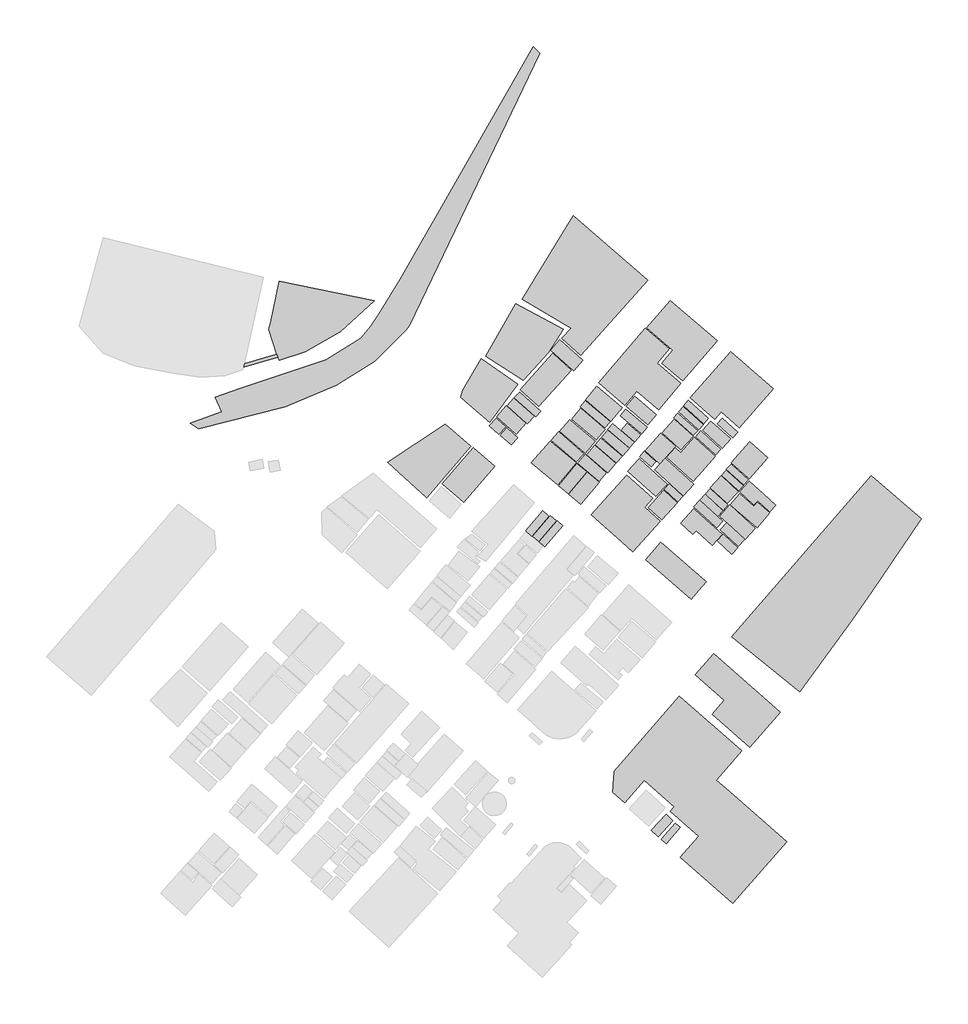
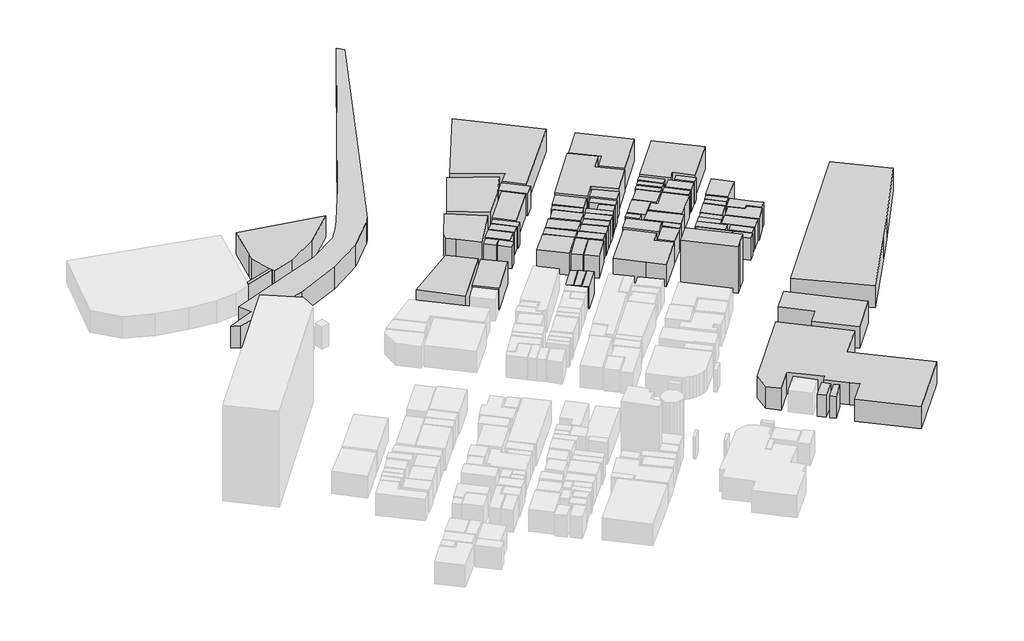
# Not in any storey, part 3 of 3: 71 proxies.
"""IFC4 building model written with IfcOpenShell, lengths in millimetres."""

from ifc_helpers import new_model, si_unit, origin, origin_with_axes, place, context, project, spatial, polyline, outline, extrude, element, save

model = new_model("IFC4")

# Units and contexts
model_context = context("Model", 3, world=origin())
ifc_project = project(units=[si_unit("LENGTHUNIT", "METRE", prefix="MILLI")], contexts=[model_context])

# Site, building
site = spatial("IfcSite", under=ifc_project)
building = spatial("IfcBuilding", under=site)

# Proxies
placement = place(None, origin())
element("IfcBuildingElementProxy", 1, Name="Mass", at=placement, inside=building, context=model_context, shape_type="SweptSolid", body=[
    extrude(outline(polyline([(247570.5222327, 178356.6623379), (255926.1515654, 187930.5455225), (280776.244849, 166225.2958414), (276476.4831621, 161299.3605912), (272420.6155188, 156651.4126569), (247570.5222327, 178356.6623379)])), origin_with_axes(), (0.0, 0.0, 1.0), 32000.0),
])
element("IfcBuildingElementProxy", 2, Name="Mass", at=placement, inside=building, context=model_context, shape_type="SweptSolid", body=[
    extrude(outline(polyline([(258708.3503039, 38751.4319358), (262511.2907886, 35271.0307322), (254408.5886169, 26397.6755858), (250596.6150174, 29878.0767893), (258708.3503039, 38751.4319358)])), origin_with_axes(), (0.0, 0.0, 1.0), 15000.0),
])
element("IfcBuildingElementProxy", 3, Name="Mass", at=placement, inside=building, context=model_context, shape_type="SweptSolid", body=[
    extrude(outline(polyline([(263766.8934663, 33847.7356711), (266413.5955132, 31557.1201823), (258708.3503039, 22661.5260503), (256061.6482569, 24952.1415391), (263766.8934663, 33847.7356711)])), origin_with_axes(), (0.0, 0.0, 1.0), 15000.0),
])
element("IfcBuildingElementProxy", 4, Name="Mass", at=placement, inside=building, context=model_context, shape_type="SweptSolid", body=[
    extrude(outline(polyline([(288409.2251578, 194680.0775697), (291896.0066931, 198527.4220315), (301913.7287781, 189453.9160172), (298426.9472428, 185595.4520625), (288409.2251578, 194680.0775697)])), origin_with_axes(), (0.0, 0.0, 1.0), 15000.0),
])
element("IfcBuildingElementProxy", 5, Name="Mass", at=placement, inside=building, context=model_context, shape_type="SweptSolid", body=[
    extrude(outline(polyline([(293955.5564102, 208390.4120248), (299230.8942796, 214483.894005), (306909.0401522, 207712.1229722), (308869.2256268, 209891.5435347), (315571.795317, 204165.0048127), (308643.3978076, 195803.1463285), (293955.5564102, 208390.4120248)])), origin_with_axes(), (0.0, 0.0, 1.0), 15000.0),
])
element("IfcBuildingElementProxy", 6, Name="Mass", at=placement, inside=building, context=model_context, shape_type="SweptSolid", body=[
    extrude(outline(polyline([(288056.9337594, 202308.0495374), (293585.1987872, 208412.6510104), (307613.6229491, 195703.0708949), (302085.3579212, 189598.4694219), (288056.9337594, 202308.0495374)])), origin_with_axes(), (0.0, 0.0, 1.0), 15000.0),
])
element("IfcBuildingElementProxy", 7, Name="Mass", at=placement, inside=building, context=model_context, shape_type="SweptSolid", body=[
    extrude(outline(polyline([(266016.138551, 103344.5648239), (300152.2717833, 73566.5634681), (286159.9800731, 57532.2550459), (291381.1192664, 52984.3825467), (324812.6697019, 23806.8337947), (295283.4239911, -10040.9018756), (266521.992868, 15055.7930682), (276621.0129658, 26631.1849313), (272176.7214726, 30511.8878715), (260912.4298247, 40330.3998944), (263188.7742487, 42943.4806703), (246667.2109559, 57354.3431635), (236026.2040895, 45156.2597103), (229459.1310908, 50882.798433), (230190.813227, 62280.2784138), (266016.138551, 103344.5648239)])), origin_with_axes(), (0.0, 0.0, 1.0), 15000.0),
])
element("IfcBuildingElementProxy", 8, Name="Mass", at=placement, inside=building, context=model_context, shape_type="SweptSolid", body=[
    extrude(outline(polyline([(286801.3310816, 188664.4320382), (290098.4172494, 192300.5061393), (298155.9538572, 185006.1189515), (294858.8676895, 181370.0448504), (286801.3310816, 188664.4320382)])), origin_with_axes(), (0.0, 0.0, 1.0), 15000.0),
])
element("IfcBuildingElementProxy", 9, Name="Mass", at=placement, inside=building, context=model_context, shape_type="SweptSolid", body=[
    extrude(outline(polyline([(371125.4389763, 224313.5255207), (398784.8303376, 200773.5595499), (371414.4985838, 160754.5054506), (360818.6572812, 145454.0835441), (332129.4910613, 105879.809151), (294768.5365618, 136180.4266618), (371125.4389763, 224313.5255207)])), origin_with_axes(), (0.0, 0.0, 1.0), 15000.0),
])
element("IfcBuildingElementProxy", 10, Name="Mass", at=placement, inside=building, context=model_context, shape_type="SweptSolid", body=[
    extrude(outline(polyline([(45355.2593164, 291052.7204921), (45843.0474089, 289418.1550711), (26927.7092252, 283791.6917827), (27442.5966544, 285726.483506), (45355.2593164, 291052.7204921)])), origin_with_axes(), (0.0, 0.0, 1.0), 15000.0),
])
element("IfcBuildingElementProxy", 11, Name="Mass", at=placement, inside=building, context=model_context, shape_type="SweptSolid", body=[
    extrude(outline(polyline([(321479.4510826, 94793.6749646), (304650.7619527, 75568.0721482), (284028.1654554, 93615.0087426), (290640.4040154, 101176.2637543), (274678.8937157, 115153.4660333), (284895.3442831, 126817.8138387), (321479.4510826, 94793.6749646)])), origin_with_axes(), (0.0, 0.0, 1.0), 15000.0),
])
element("IfcBuildingElementProxy", 12, Name="Mass", at=placement, inside=building, context=model_context, shape_type="SweptSolid", body=[
    extrude(outline(polyline([(157465.2221542, 288561.9541354), (177428.401421, 274562.5128708), (162045.010339, 253624.5081838), (150672.3213364, 263331.8252796), (146237.0629554, 267490.5155365), (147212.6391378, 271371.2184759), (157465.2221542, 288561.9541354)])), origin_with_axes(), (0.0, 0.0, 1.0), 15000.0),
])
element("IfcBuildingElementProxy", 13, Name="Mass", at=placement, inside=building, context=model_context, shape_type="SweptSolid", body=[
    extrude(outline(polyline([(41913.6433449, 308488.0849906), (46646.9944457, 331171.8500257), (98713.8565671, 320363.703156), (80105.6442205, 303306.4014085), (60720.5841739, 292442.6570756), (46728.2924611, 287872.54559), (45843.0474089, 289418.1550711), (45355.2593164, 291052.7204921), (40929.0340502, 304629.621036), (41913.6433449, 308488.0849906)])), origin_with_axes(), (0.0, 0.0, 1.0), 15000.0),
])
element("IfcBuildingElementProxy", 14, Name="Mass", at=placement, inside=building, context=model_context, shape_type="SweptSolid", body=[
    extrude(outline(polyline([(175314.6530278, 266967.8993815), (186371.183081, 257071.5509098), (182640.5074995, 252912.8606537), (171583.9774437, 262798.0896318), (175314.6530278, 266967.8993815)])), origin_with_axes(), (0.0, 0.0, 1.0), 15000.0),
])
element("IfcBuildingElementProxy", 15, Name="Mass", at=placement, inside=building, context=model_context, shape_type="SweptSolid", body=[
    extrude(outline(polyline([(236640.4557587, 260996.7318204), (248347.3699327, 251078.1443639), (245312.2440357, 247497.667726), (233605.3298618, 257427.3746753), (236640.4557587, 260996.7318204)])), origin_with_axes(), (0.0, 0.0, 1.0), 15000.0),
])
element("IfcBuildingElementProxy", 16, Name="Mass", at=placement, inside=building, context=model_context, shape_type="SweptSolid", body=[
    extrude(outline(polyline([(199803.4218007, 248465.0635873), (213461.4883396, 236578.3259291), (209486.9187118, 231997.0949516), (195819.8190607, 243883.8326097), (199803.4218007, 248465.0635873)])), origin_with_axes(), (0.0, 0.0, 1.0), 15000.0),
])
element("IfcBuildingElementProxy", 17, Name="Mass", at=placement, inside=building, context=model_context, shape_type="SweptSolid", body=[
    extrude(outline(polyline([(178458.176277, 270237.0302243), (190029.593762, 259873.6630616), (187184.1632327, 256693.4881595), (175603.7126354, 267045.7358294), (178458.176277, 270237.0302243)])), origin_with_axes(), (0.0, 0.0, 1.0), 15000.0),
])
element("IfcBuildingElementProxy", 18, Name="Mass", at=placement, inside=building, context=model_context, shape_type="SweptSolid", body=[
    extrude(outline(polyline([(237408.2703439, 253190.8479696), (244743.1579304, 246975.0515702), (241464.1379872, 243116.5876156), (234129.2504033, 249332.384015), (237408.2703439, 253190.8479696)])), origin_with_axes(), (0.0, 0.0, 1.0), 15000.0),
])
element("IfcBuildingElementProxy", 19, Name="Mass", at=placement, inside=building, context=model_context, shape_type="SweptSolid", body=[
    extrude(outline(polyline([(220805.4090383, 273361.6076632), (234608.005381, 261652.7818874), (228402.256893, 254325.036222), (214599.6605503, 266033.861997), (220805.4090383, 273361.6076632)])), origin_with_axes(), (0.0, 0.0, 1.0), 15000.0),
])
element("IfcBuildingElementProxy", 20, Name="Mass", at=placement, inside=building, context=model_context, shape_type="SweptSolid", body=[
    extrude(outline(polyline([(214491.2631982, 265411.1704084), (228022.8661552, 253935.8539781), (225222.6011923, 250622.2451641), (211681.9651204, 262108.6810864), (214491.2631982, 265411.1704084)])), origin_with_axes(), (0.0, 0.0, 1.0), 15000.0),
])
element("IfcBuildingElementProxy", 21, Name="Mass", at=placement, inside=building, context=model_context, shape_type="SweptSolid", body=[
    extrude(outline(polyline([(171051.0237899, 262709.133691), (181782.361784, 253101.8920288), (176507.0239146, 247208.5609165), (165775.6859206, 256815.8025787), (171051.0237899, 262709.133691)])), origin_with_axes(), (0.0, 0.0, 1.0), 15000.0),
])
element("IfcBuildingElementProxy", 22, Name="Mass", at=placement, inside=building, context=model_context, shape_type="SweptSolid", body=[
    extrude(outline(polyline([(207029.9120325, 255370.268532), (212061.3558556, 261296.9581227), (225394.2303353, 249988.4340827), (220371.8196245, 244061.7444921), (207029.9120325, 255370.268532)])), origin_with_axes(), (0.0, 0.0, 1.0), 15000.0),
])
element("IfcBuildingElementProxy", 23, Name="Mass", at=placement, inside=building, context=model_context, shape_type="SweptSolid", body=[
    extrude(outline(polyline([(247236.2970613, 238123.9354094), (255890.0191138, 247797.8940275), (263911.4232701, 240614.7017661), (255266.7343298, 230951.8626407), (247236.2970613, 238123.9354094)])), origin_with_axes(), (0.0, 0.0, 1.0), 15000.0),
])
element("IfcBuildingElementProxy", 24, Name="Mass", at=placement, inside=building, context=model_context, shape_type="SweptSolid", body=[
    extrude(outline(polyline([(214355.7665041, 236055.7097741), (226008.4820045, 226159.3613024), (222033.9123767, 221478.0548905), (210381.1968788, 231374.4033622), (214355.7665041, 236055.7097741)])), origin_with_axes(), (0.0, 0.0, 1.0), 15000.0),
])
element("IfcBuildingElementProxy", 25, Name="Mass", at=placement, inside=building, context=model_context, shape_type="SweptSolid", body=[
    extrude(outline(polyline([(288942.1788116, 259417.7638618), (285500.5628401, 255503.702444), (272122.5227965, 267268.125683), (294280.7484718, 292476.0155532), (317595.2125825, 271982.7905725), (298878.6028811, 250688.9621201), (288942.1788116, 259417.7638618)])), origin_with_axes(), (0.0, 0.0, 1.0), 15000.0),
])
element("IfcBuildingElementProxy", 26, Name="Mass", at=placement, inside=building, context=model_context, shape_type="SweptSolid", body=[
    extrude(outline(polyline([(260912.4298247, 320497.137068), (286683.9006146, 298558.3780406), (267822.7611095, 276397.2291605), (256441.0389947, 286082.3072714), (262502.2576763, 293209.9020689), (248112.5090013, 305452.4634925), (260912.4298247, 320497.137068)])), origin_with_axes(), (0.0, 0.0, 1.0), 15000.0),
])
element("IfcBuildingElementProxy", 27, Name="Mass", at=placement, inside=building, context=model_context, shape_type="SweptSolid", body=[
    extrude(outline(polyline([(259042.5754778, 234465.6223227), (263703.661678, 239680.6643824), (266684.5888963, 237011.9861434), (274164.0062865, 245373.8446268), (285717.357547, 235032.7164489), (278237.9401568, 226681.9774575), (273567.8208444, 221466.9353985), (259042.5754778, 234465.6223227)])), origin_with_axes(), (0.0, 0.0, 1.0), 15000.0),
])
element("IfcBuildingElementProxy", 28, Name="Mass", at=placement, inside=building, context=model_context, shape_type="SweptSolid", body=[
    extrude(outline(polyline([(242530.0452973, 270815.2438433), (236017.1709747, 263142.7939044), (221690.6540905, 275318.6383721), (247191.1314975, 305330.1490734), (260524.0059747, 293999.3860486), (253830.4693967, 286115.665749), (266919.4498303, 275007.2925778), (254625.3833238, 260529.7131286), (242530.0452973, 270815.2438433)])), origin_with_axes(), (0.0, 0.0, 1.0), 15000.0),
])
element("IfcBuildingElementProxy", 29, Name="Mass", at=placement, inside=building, context=model_context, shape_type="SweptSolid", body=[
    extrude(outline(polyline([(217788.3493659, 203008.5775755), (237236.6412034, 224747.1857341), (251454.7607328, 212026.4861259), (246947.2374512, 206989.3559493), (255474.4959245, 199361.3839816), (240533.7273711, 182659.9059996), (232006.4688979, 190287.8779672), (217788.3493659, 203008.5775755)])), origin_with_axes(), (0.0, 0.0, 1.0), 15000.0),
])
element("IfcBuildingElementProxy", 30, Name="Mass", at=placement, inside=building, context=model_context, shape_type="SweptSolid", body=[
    extrude(outline(polyline([(257660.5092208, 216885.7044202), (260352.3768316, 219899.0869327), (267958.2578011, 213093.9574215), (265266.3901903, 210080.5749098), (257660.5092208, 216885.7044202)])), origin_with_axes(), (0.0, 0.0, 1.0), 15000.0),
])
element("IfcBuildingElementProxy", 31, Name="Mass", at=placement, inside=building, context=model_context, shape_type="SweptSolid", body=[
    extrude(outline(polyline([(252394.2044637, 227560.4173779), (258157.330423, 234009.7231236), (273965.2778066, 219865.7284543), (268202.1518473, 213416.4227094), (252394.2044637, 227560.4173779)])), origin_with_axes(), (0.0, 0.0, 1.0), 15000.0),
])
element("IfcBuildingElementProxy", 32, Name="Mass", at=placement, inside=building, context=model_context, shape_type="SweptSolid", body=[
    extrude(outline(polyline([(237814.760421, 226748.6944142), (243939.2108936, 233587.1824022), (259286.4695215, 219865.7284543), (253162.0190515, 213016.1209735), (237814.760421, 226748.6944142)])), origin_with_axes(), (0.0, 0.0, 1.0), 15000.0),
])
element("IfcBuildingElementProxy", 33, Name="Mass", at=placement, inside=building, context=model_context, shape_type="SweptSolid", body=[
    extrude(outline(polyline([(176416.692787, 318662.4207782), (202441.0907354, 304763.054948), (194022.2296144, 291819.9654862), (180454.4942031, 276842.0088675), (159849.9639304, 289985.2491965), (176416.692787, 318662.4207782)])), origin_with_axes(), (0.0, 0.0, 1.0), 15000.0),
])
element("IfcBuildingElementProxy", 34, Name="Mass", at=placement, inside=building, context=model_context, shape_type="SweptSolid", body=[
    extrude(outline(polyline([(277686.9202759, 248943.2017719), (288761.5165562, 239046.853301), (285979.3178178, 235933.395355), (274913.7546497, 245840.8633186), (277686.9202759, 248943.2017719)])), origin_with_axes(), (0.0, 0.0, 1.0), 15000.0),
])
element("IfcBuildingElementProxy", 35, Name="Mass", at=placement, inside=building, context=model_context, shape_type="SweptSolid", body=[
    extrude(outline(polyline([(270975.3174735, 265733.6356955), (281896.3508352, 255959.601643), (279267.7150128, 253024.05558), (268346.6816511, 262798.0896318), (270975.3174735, 265733.6356955)])), origin_with_axes(), (0.0, 0.0, 1.0), 15000.0),
])
element("IfcBuildingElementProxy", 36, Name="Mass", at=placement, inside=building, context=model_context, shape_type="SweptSolid", body=[
    extrude(outline(polyline([(223325.647506, 245485.0395531), (226667.8992376, 249421.3399565), (238456.1114295, 239424.9160513), (235113.8596954, 235488.6156479), (223325.647506, 245485.0395531)])), origin_with_axes(), (0.0, 0.0, 1.0), 15000.0),
])
element("IfcBuildingElementProxy", 37, Name="Mass", at=placement, inside=building, context=model_context, shape_type="SweptSolid", body=[
    extrude(outline(polyline([(205394.918617, 214194.7871955), (215484.9056051, 226337.2731856), (222061.011716, 220877.6022867), (211961.9916156, 208735.1162975), (205394.918617, 214194.7871955)])), origin_with_axes(), (0.0, 0.0, 1.0), 15000.0),
])
element("IfcBuildingElementProxy", 38, Name="Mass", at=placement, inside=building, context=model_context, shape_type="SweptSolid", body=[
    extrude(outline(polyline([(244210.2042766, 234910.4020297), (246721.409632, 237712.5141807), (252990.3899084, 232108.2898779), (250479.1845529, 229306.1777269), (244210.2042766, 234910.4020297)])), origin_with_axes(), (0.0, 0.0, 1.0), 15000.0),
])
element("IfcBuildingElementProxy", 39, Name="Mass", at=placement, inside=building, context=model_context, shape_type="SweptSolid", body=[
    extrude(outline(polyline([(219865.9653075, 241315.2298042), (223045.6210082, 245062.4988325), (234644.1378325, 235221.747824), (231473.5152415, 231485.5982885), (219865.9653075, 241315.2298042)])), origin_with_axes(), (0.0, 0.0, 1.0), 15000.0),
])
element("IfcBuildingElementProxy", 40, Name="Mass", at=placement, inside=building, context=model_context, shape_type="SweptSolid", body=[
    extrude(outline(polyline([(268175.052508, 262130.920072), (279150.2845483, 252312.4080491), (276684.2447567, 249554.7738685), (265709.0127164, 259373.2858914), (268175.052508, 262130.920072)])), origin_with_axes(), (0.0, 0.0, 1.0), 15000.0),
])
element("IfcBuildingElementProxy", 41, Name="Mass", at=placement, inside=building, context=model_context, shape_type="SweptSolid", body=[
    extrude(outline(polyline([(200381.5410184, 248687.4534408), (205828.5080308, 255103.4007081), (219874.9984197, 243194.4240644), (214428.0314072, 236778.4767971), (200381.5410184, 248687.4534408)])), origin_with_axes(), (0.0, 0.0, 1.0), 15000.0),
])
element("IfcBuildingElementProxy", 42, Name="Mass", at=placement, inside=building, context=model_context, shape_type="SweptSolid", body=[
    extrude(outline(polyline([(165513.7256498, 255970.7211358), (170807.1297437, 251233.8172607), (167058.3879376, 247041.7685262), (161764.9838411, 251789.7918941), (165513.7256498, 255970.7211358)])), origin_with_axes(), (0.0, 0.0, 1.0), 15000.0),
])
element("IfcBuildingElementProxy", 43, Name="Mass", at=placement, inside=building, context=model_context, shape_type="SweptSolid", body=[
    extrude(outline(polyline([(199767.2893492, 218953.9300562), (209766.9452071, 230951.8626407), (215141.6473189, 226470.7070975), (205141.9914585, 214472.7745122), (199767.2893492, 218953.9300562)])), origin_with_axes(), (0.0, 0.0, 1.0), 15000.0),
])
element("IfcBuildingElementProxy", 44, Name="Mass", at=placement, inside=building, context=model_context, shape_type="SweptSolid", body=[
    extrude(outline(polyline([(226685.9654646, 249855.0001708), (229368.7999632, 253012.9360873), (241346.7075227, 242860.8392845), (238663.8730242, 239691.7838752), (226685.9654646, 249855.0001708)])), origin_with_axes(), (0.0, 0.0, 1.0), 15000.0),
])
element("IfcBuildingElementProxy", 45, Name="Mass", at=placement, inside=building, context=model_context, shape_type="SweptSolid", body=[
    extrude(outline(polyline([(241608.6677935, 267990.8927059), (253414.94621, 257983.3493087), (248708.6944459, 252434.7224691), (236902.4160295, 262442.2658671), (241608.6677935, 267990.8927059)])), origin_with_axes(), (0.0, 0.0, 1.0), 15000.0),
])
element("IfcBuildingElementProxy", 46, Name="Mass", at=placement, inside=building, context=model_context, shape_type="SweptSolid", body=[
    extrude(outline(polyline([(265266.3901903, 258717.2358244), (276006.7612966, 249109.9941622), (273730.4168726, 246563.6303416), (262990.0457663, 256181.9914965), (265266.3901903, 258717.2358244)])), origin_with_axes(), (0.0, 0.0, 1.0), 15000.0),
])
element("IfcBuildingElementProxy", 47, Name="Mass", at=placement, inside=building, context=model_context, shape_type="SweptSolid", body=[
    extrude(outline(polyline([(200562.2032737, 298903.0823133), (213109.1969412, 287683.5142149), (207969.3557633, 281934.7365073), (195422.3620984, 293165.4240985), (200562.2032737, 298903.0823133)])), origin_with_axes(), (0.0, 0.0, 1.0), 15000.0),
])
element("IfcBuildingElementProxy", 48, Name="Mass", at=placement, inside=building, context=model_context, shape_type="SweptSolid", body=[
    extrude(outline(polyline([(215123.5810919, 235900.0368766), (219513.673909, 241070.6009659), (231039.9258277, 231307.6864062), (226649.8330131, 226126.0028249), (215123.5810919, 235900.0368766)])), origin_with_axes(), (0.0, 0.0, 1.0), 15000.0),
])
element("IfcBuildingElementProxy", 49, Name="Mass", at=placement, inside=building, context=model_context, shape_type="SweptSolid", body=[
    extrude(outline(polyline([(263188.7742487, 255303.551576), (273558.7877295, 246029.8946938), (266910.416718, 238590.9541012), (256540.4032346, 247875.7304763), (263188.7742487, 255303.551576)])), origin_with_axes(), (0.0, 0.0, 1.0), 15000.0),
])
element("IfcBuildingElementProxy", 50, Name="Mass", at=placement, inside=building, context=model_context, shape_type="SweptSolid", body=[
    extrude(outline(polyline([(289565.4635956, 255881.765195), (298065.6227295, 248276.0322121), (295364.7220065, 245262.6497004), (286864.56287, 252868.3826825), (289565.4635956, 255881.765195)])), origin_with_axes(), (0.0, 0.0, 1.0), 15000.0),
])
element("IfcBuildingElementProxy", 51, Name="Mass", at=placement, inside=building, context=model_context, shape_type="SweptSolid", body=[
    extrude(outline(polyline([(249042.9196199, 206900.4000077), (257452.7476261, 216307.490802), (264868.933228, 209669.1536811), (256459.1052192, 200273.1823797), (249042.9196199, 206900.4000077)])), origin_with_axes(), (0.0, 0.0, 1.0), 15000.0),
])
element("IfcBuildingElementProxy", 52, Name="Mass", at=placement, inside=building, context=model_context, shape_type="SweptSolid", body=[
    extrude(outline(polyline([(195332.0309707, 243361.2164547), (209351.4220203, 231652.3906789), (199198.2032438, 219498.7851968), (184781.355232, 231641.2711861), (195332.0309707, 243361.2164547)])), origin_with_axes(), (0.0, 0.0, 1.0), 15000.0),
])
element("IfcBuildingElementProxy", 53, Name="Mass", at=placement, inside=building, context=model_context, shape_type="SweptSolid", body=[
    extrude(outline(polyline([(283323.582656, 254369.5141924), (294253.6491325, 244584.3606479), (289673.8609478, 239458.2745297), (278734.761359, 249243.4280742), (283323.582656, 254369.5141924)])), origin_with_axes(), (0.0, 0.0, 1.0), 15000.0),
])
element("IfcBuildingElementProxy", 54, Name="Mass", at=placement, inside=building, context=model_context, shape_type="SweptSolid", body=[
    extrude(outline(polyline([(178674.9709839, 271682.564271), (196470.2031814, 291564.2171551), (206840.2166649, 282279.44078), (189044.9844673, 262397.7878959), (178674.9709839, 271682.564271)])), origin_with_axes(), (0.0, 0.0, 1.0), 15000.0),
])
element("IfcBuildingElementProxy", 55, Name="Mass", at=placement, inside=building, context=model_context, shape_type="SweptSolid", body=[
    extrude(outline(polyline([(289240.2715339, 224658.2297926), (291778.5762287, 227449.2224516), (301109.7817413, 218998.4080266), (298571.4770465, 216196.2958756), (289240.2715339, 224658.2297926)])), origin_with_axes(), (0.0, 0.0, 1.0), 15000.0),
])
element("IfcBuildingElementProxy", 56, Name="Mass", at=placement, inside=building, context=model_context, shape_type="SweptSolid", body=[
    extrude(outline(polyline([(185720.7989603, 191288.6323069), (195332.0309707, 202530.4393909), (198475.5542199, 199850.6416582), (188864.322212, 188597.7150823), (185720.7989603, 191288.6323069)])), origin_with_axes(), (0.0, 0.0, 1.0), 15000.0),
])
element("IfcBuildingElementProxy", 57, Name="Mass", at=placement, inside=building, context=model_context, shape_type="SweptSolid", body=[
    extrude(outline(polyline([(181782.361784, 194168.5809067), (191122.6004089, 205087.9227036), (194455.8190282, 202241.3325814), (185115.5804033, 191321.9907845), (181782.361784, 194168.5809067)])), origin_with_axes(), (0.0, 0.0, 1.0), 15000.0),
])
element("IfcBuildingElementProxy", 58, Name="Mass", at=placement, inside=building, context=model_context, shape_type="SweptSolid", body=[
    extrude(outline(polyline([(179894.4412126, 321264.3820621), (207897.0908602, 367032.2138689), (248699.6613337, 331672.227196), (211862.6273757, 290596.821293), (201546.8125684, 299903.8366529), (206641.4881824, 305407.9855221), (179894.4412126, 321264.3820621)])), origin_with_axes(), (0.0, 0.0, 1.0), 15000.0),
])
element("IfcBuildingElementProxy", 59, Name="Mass", at=placement, inside=building, context=model_context, shape_type="SweptSolid", body=[
    extrude(outline(polyline([(308950.5236422, 210614.3105576), (306954.205716, 208412.6510104), (299113.4638126, 215518.006823), (304325.5698936, 221277.9040226), (312175.3449067, 214172.5482107), (318814.6828086, 208156.9026785), (315589.8615415, 204598.6650261), (308950.5236422, 210614.3105576)])), origin_with_axes(), (0.0, 0.0, 1.0), 15000.0),
])
element("IfcBuildingElementProxy", 60, Name="Mass", at=placement, inside=building, context=model_context, shape_type="SweptSolid", body=[
    extrude(outline(polyline([(274010.4433705, 206311.0668967), (280631.7150452, 200306.5408581), (289520.2980317, 192256.0281689), (284127.5296954, 186307.0995935), (275247.9798237, 194357.6122826), (273405.2248135, 192322.7451249), (266774.9200265, 198327.2711636), (274010.4433705, 206311.0668967)])), origin_with_axes(), (0.0, 0.0, 1.0), 15000.0),
])
element("IfcBuildingElementProxy", 61, Name="Mass", at=placement, inside=building, context=model_context, shape_type="SweptSolid", body=[
    extrude(outline(polyline([(273802.6817758, 207456.3746411), (277090.7348313, 211081.3292494), (289890.6556547, 199483.6984008), (286602.6025992, 195858.7437917), (273802.6817758, 207456.3746411)])), origin_with_axes(), (0.0, 0.0, 1.0), 15000.0),
])
element("IfcBuildingElementProxy", 62, Name="Mass", at=placement, inside=building, context=model_context, shape_type="SweptSolid", body=[
    extrude(outline(polyline([(291868.9073563, 227882.8826658), (294371.0795995, 230640.5168464), (303738.4175612, 222145.2244511), (301245.2784328, 219387.5902697), (291868.9073563, 227882.8826658)])), origin_with_axes(), (0.0, 0.0, 1.0), 15000.0),
])
element("IfcBuildingElementProxy", 63, Name="Mass", at=placement, inside=building, context=model_context, shape_type="SweptSolid", body=[
    extrude(outline(polyline([(282953.2250331, 217741.9053558), (288878.9470232, 224280.1670423), (298291.4505487, 215751.5161686), (292365.7285585, 209213.2544821), (282953.2250331, 217741.9053558)])), origin_with_axes(), (0.0, 0.0, 1.0), 15000.0),
])
element("IfcBuildingElementProxy", 64, Name="Mass", at=placement, inside=building, context=model_context, shape_type="SweptSolid", body=[
    extrude(outline(polyline([(294461.4107272, 231596.7932157), (304741.0930829, 243060.9901524), (314578.15291, 234254.351962), (304298.4705543, 222779.0355325), (294461.4107272, 231596.7932157)])), origin_with_axes(), (0.0, 0.0, 1.0), 15000.0),
])
element("IfcBuildingElementProxy", 65, Name="Mass", at=placement, inside=building, context=model_context, shape_type="SweptSolid", body=[
    extrude(outline(polyline([(277253.3308621, 211025.7317862), (280125.8607282, 214194.7871955), (289935.8212185, 205310.3125571), (287063.2913524, 202141.257147), (277253.3308621, 211025.7317862)])), origin_with_axes(), (0.0, 0.0, 1.0), 15000.0),
])
element("IfcBuildingElementProxy", 66, Name="Mass", at=placement, inside=building, context=model_context, shape_type="SweptSolid", body=[
    extrude(outline(polyline([(280243.2911952, 214172.5482107), (282953.2250331, 217163.6917369), (292672.8543931, 208357.0535472), (289962.9205578, 205365.9100203), (280243.2911952, 214172.5482107)])), origin_with_axes(), (0.0, 0.0, 1.0), 15000.0),
])
element("IfcBuildingElementProxy", 67, Name="Mass", at=placement, inside=building, context=model_context, shape_type="SweptSolid", body=[
    extrude(outline(polyline([(127520.453254, 212393.4293842), (106157.1415058, 231663.5101717), (137592.3740151, 252757.1877561), (151738.2286439, 240625.8212589), (127520.453254, 212393.4293842)])), origin_with_axes(), (0.0, 0.0, 1.0), 15000.0),
])
element("IfcBuildingElementProxy", 68, Name="Mass", at=placement, inside=building, context=model_context, shape_type="SweptSolid", body=[
    extrude(outline(polyline([(135993.5130512, 219965.8038887), (152948.6657578, 239736.2618456), (164718.8117253, 229650.8819996), (147763.6590187, 209880.4240419), (135993.5130512, 219965.8038887)])), origin_with_axes(), (0.0, 0.0, 1.0), 15000.0),
])
element("IfcBuildingElementProxy", 69, Name="Mass", at=placement, inside=building, context=model_context, shape_type="SweptSolid", body=[
    extrude(outline(polyline([(189135.315595, 188152.9353752), (198954.3091975, 199639.3712975), (202124.9317886, 196926.2150881), (192314.9712983, 185439.779165), (189135.315595, 188152.9353752)])), origin_with_axes(), (0.0, 0.0, 1.0), 15000.0),
])
element("IfcBuildingElementProxy", 70, Name="Mass", at=placement, inside=building, context=model_context, shape_type="SweptSolid", body=[
    extrude(outline(polyline([(14949.8016656, 259362.1663986), (11481.0863548, 267457.1570581), (24777.828383, 272082.8660068), (72337.1672202, 288128.2939219), (91279.6047407, 299692.566293), (96816.9028809, 306342.0229058), (101107.6314581, 312991.4795194), (112959.0754384, 332217.0823366), (186009.8585704, 459779.902183), (189334.0440774, 455965.9161988), (117855.0225701, 306653.3687009), (115949.0357716, 304162.6023434), (99084.2141926, 287260.9734934), (77829.2997965, 274106.6136717), (49935.0475012, 262253.2344912), (2375.7086639, 250255.3019066), (-2113.7483932, 253146.3699992), (14949.8016656, 259362.1663986)])), origin_with_axes(), (0.0, 0.0, 1.0), 15000.0),
])
element("IfcBuildingElementProxy", 71, Name="Mass", at=placement, inside=building, context=model_context, shape_type="SweptSolid", body=[
    extrude(outline(polyline([(171448.4807522, 250722.3205985), (177527.7656609, 245273.7691924), (173959.6861076, 241281.8713266), (167871.3680892, 246719.3032391), (171448.4807522, 250722.3205985)])), origin_with_axes(), (0.0, 0.0, 1.0), 15000.0),
])

save(model, "model.ifc")

# Revit data of these elements
# Elements 1, 2, 3, 4, 5, 6, 7, 8, 9, 10, 11, 12, 13, 14, 15, 16, 17, 18, 19, 20, 21, 22, 23, 24, 25, 26, 27, 28, 29, 30, 31, 32, 33, 34, 35, 36, 37, 38, 39, 40, 41, 42, 43, 44, 45, 46, 47, 48, 49, 50, 51, 52, 53, 54, 55, 56, 57, 58, 59, 60, 61, 62, 63, 64, 65, 66, 67, 68, 69, 70, 71 (IfcBuildingElementProxy)
#   Phase Created = 新しい建設
#   Materials on its faces: "周辺建物"
# Materials
#   "周辺建物": class "一般", colour RGB 120 120 120, transparency 0, Cost = 0
